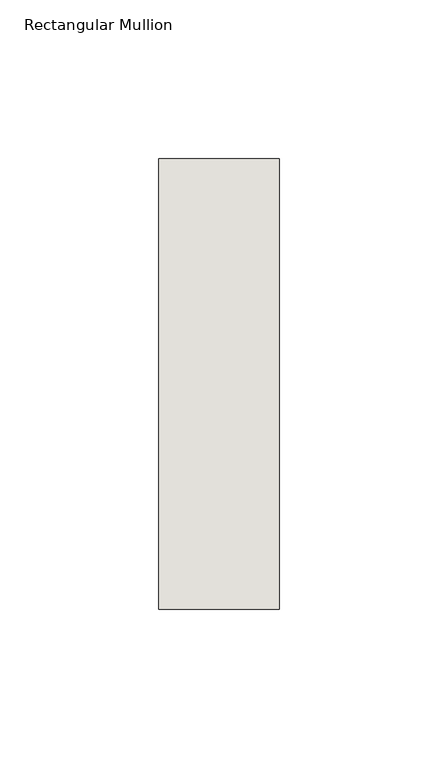
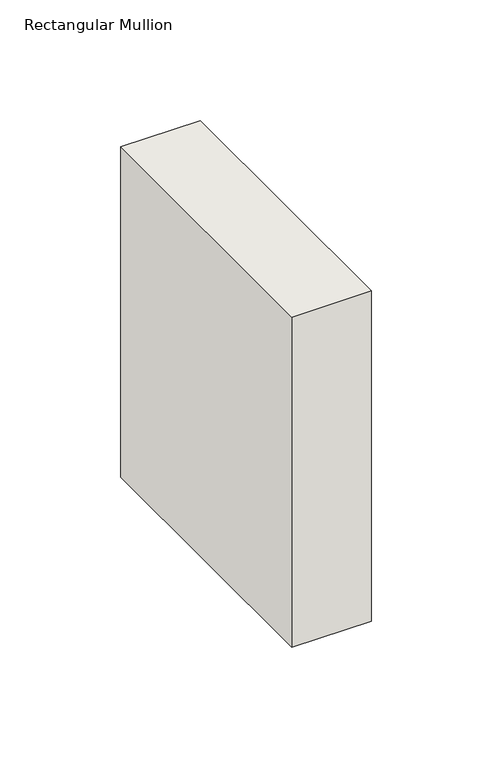
"""IFC4 building model written with IfcOpenShell, lengths in millimetres: wall geometry, Rectangular Mullion : NLRS_21_CWM_hsb-regel 38x142_gen_rsf."""

from ifc_helpers import new_model, si_unit, frame, origin, place, context, project, spatial, polyline, outline, extrude, source, transform, mapped, element, save


def rectangular_mullion_f999a466(model_context):
    return source(origin(), model_context, "Body", "SweptSolid", [
        extrude(outline(polyline([(0.0, -71.0), (-38.0, -71.0), (-38.0, 71.0), (0.0, 71.0), (0.0, -71.0)])), frame((0.0, 0.0, -167.1558939), z_axis=(0.0, 0.0, 1.0), x_axis=(1.0, 0.0, 0.0)), (0.0, 0.0, 1.0), 167.1558939),
    ])


if __name__ == "__main__":
    model = new_model("IFC4")
    model_context = context("Model", 3, world=origin())
    ifc_project = project(units=[si_unit("LENGTHUNIT", "METRE", prefix="MILLI")], contexts=[model_context])
    site = spatial("IfcSite", under=ifc_project)
    building = spatial("IfcBuilding", under=site)
    placement = place(None, origin())
    rectangular_mullion_shape = rectangular_mullion_f999a466(model_context)
    element("IfcWall", 1, ObjectType="Rectangular Mullion : NLRS_21_CWM_hsb-regel 38x142_gen_rsf", at=placement, inside=building, context=model_context, shape_type="MappedRepresentation", body=[
        mapped(rectangular_mullion_shape, transform((0.0, 0.0, 0.0), x_axis=(1.0, 0.0, 0.0), y_axis=(0.0, 1.0, 0.0), z_axis=(0.0, 0.0, 1.0))),
    ])
    save(model, "model.ifc")

# Revit data of these elements
# Type "Rectangular Mullion : NLRS_21_CWM_hsb-regel 38x142_gen_rsf"
#   Type IfcGUID = "07M7mRoiH1CR8m_RSKIwpF"
#   Assembly Code = "21.10"
#   IfcExportAs = "IfcWall"
#   built-in parameter 1007322 = 0.465879 (stored number, unit not read)
#   built-in parameter 1007321 = 0.062336 (stored number, unit not read)
#   built-in parameter 1007320 = 0.062336 (stored number, unit not read)
# Element 1 (IfcWall, "Rectangular Mullion : NLRS_21_CWM_hsb-regel 38x142_gen_rsf")
#   Materials on its faces: "NLRS_i2_hout naaldhout vuren_gen_rsf"
# Materials
#   "NLRS_i2_hout naaldhout vuren_gen_rsf": class "I - Hout", colour RGB 234 199 147, transparency 0, Keynote = "i2", Manufacturer = "Revit Standards Foundation", URL = "www.revitstandards.org", Description = "hout vuren", Cost = 0
